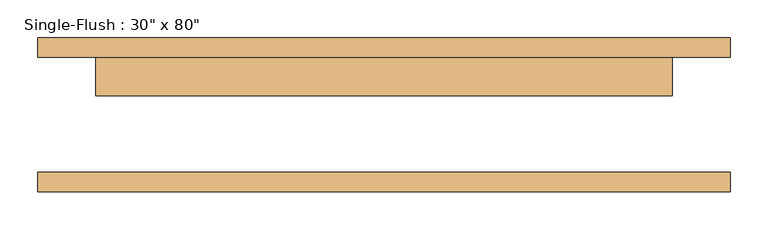
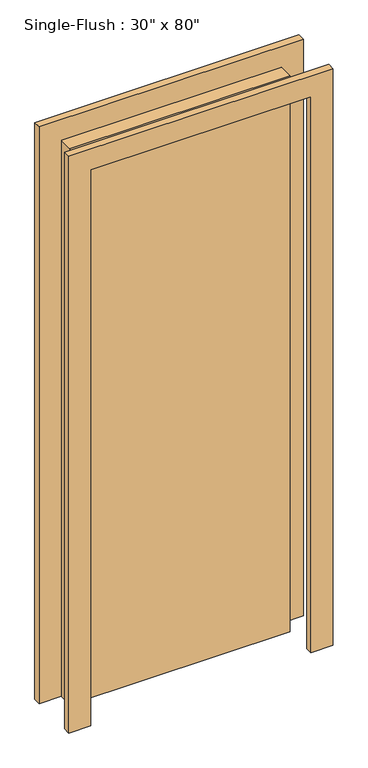
"""IFC4 building model written with IfcOpenShell, lengths in millimetres: door geometry."""

import ifcopenshell
import ifcopenshell.guid

model = None  # the IFC model being written
_history = None  # IfcOwnerHistory: only IFC2X3 demands one
_inside = {}  # id of a spatial element -> (the spatial element, [elements in it])
_under = {}  # id of a project, library or spatial element -> (it, [spatial elements below it])
_declared = {}  # id of a project -> (the project, [libraries it declares])
_typed = {}  # id of a type object -> (the type object, [elements of that type])
_made_of = {}  # id of a material, layer set ... -> (it, [elements and type objects made of it])


def new_model(schema):
    """Start an empty IFC model of exactly this schema.

    Asked for "IFC4X3", IfcOpenShell would pick the latest addendum, in which some entities
    have other attributes; the version numbers below select the first issue.
    IFC2X3 requires an IfcOwnerHistory on every rooted entity: one is made here for all.
    """
    global model, _history
    if schema == "IFC4X3":
        model = ifcopenshell.file(schema_version=(4, 3, 0, 0))
    else:
        model = ifcopenshell.file(schema=schema)
    _inside.clear()
    _under.clear()
    _declared.clear()
    _typed.clear()
    _made_of.clear()
    _history = None
    if model.schema == "IFC2X3":
        org = make("IfcOrganization", Name="unknown")
        user = make(
            "IfcPersonAndOrganization",
            ThePerson=make("IfcPerson", FamilyName="unknown"),
            TheOrganization=org,
        )
        app = make(
            "IfcApplication",
            ApplicationDeveloper=org,
            Version="unknown",
            ApplicationFullName="unknown",
            ApplicationIdentifier="unknown",
        )
        _history = make(
            "IfcOwnerHistory",
            OwningUser=user,
            OwningApplication=app,
            ChangeAction="ADDED",
            CreationDate=0,
        )
    return model


def make(cls, **values):
    """One entity of the class cls with the attributes given. An attribute that is None is left unset."""
    return model.create_entity(
        cls, **{name: value for name, value in values.items() if value is not None}
    )


def rooted(cls, **values):
    """An entity with a GlobalId (a new one), such as an element, a storey or a relation."""
    return make(cls, GlobalId=ifcopenshell.guid.new(), OwnerHistory=_history, **values)


def si_unit(unit_type, name, prefix=None):
    """IfcSIUnit, for example si_unit("LENGTHUNIT", "METRE", prefix="MILLI")."""
    return make("IfcSIUnit", UnitType=unit_type, Prefix=prefix, Name=name)


def assignment(units):
    """IfcUnitAssignment: the units of a project."""
    return None if units is None else make("IfcUnitAssignment", Units=units)


def point(xyz):
    """IfcCartesianPoint."""
    return None if xyz is None else make("IfcCartesianPoint", Coordinates=xyz)


def direction(xyz):
    """IfcDirection."""
    return None if xyz is None else make("IfcDirection", DirectionRatios=xyz)


def frame(location, z_axis=None, x_axis=None):
    """IfcAxis2Placement3D, a coordinate frame: its origin and axes. An axis left out is left unset."""
    return make(
        "IfcAxis2Placement3D",
        Location=point(location),
        Axis=direction(z_axis),
        RefDirection=direction(x_axis),
    )


def origin():
    """The frame at (0, 0, 0) with its axes left unset."""
    return frame((0.0, 0.0, 0.0))


def origin_with_axes():
    """The frame at (0, 0, 0) with the z axis (0, 0, 1) and the x axis (1, 0, 0) written out."""
    return frame((0.0, 0.0, 0.0), z_axis=(0.0, 0.0, 1.0), x_axis=(1.0, 0.0, 0.0))


def place(relative_to, where):
    """IfcLocalPlacement: puts the frame where relative to a parent placement (None: the world)."""
    return make(
        "IfcLocalPlacement", PlacementRelTo=relative_to, RelativePlacement=where
    )


def context(
    kind, dimensions, precision=None, world=None, true_north=None, identifier=None
):
    """IfcGeometricRepresentationContext, for example the 3D "Model" context."""
    return make(
        "IfcGeometricRepresentationContext",
        ContextIdentifier=identifier,
        ContextType=kind,
        CoordinateSpaceDimension=dimensions,
        Precision=precision,
        WorldCoordinateSystem=world,
        TrueNorth=true_north,
    )


def project(units=None, contexts=None):
    """IfcProject with its units and contexts."""
    return rooted(
        "IfcProject",
        Name="project",
        RepresentationContexts=contexts,
        UnitsInContext=assignment(units),
    )


def spatial(cls, under=None, at=None, **own):
    """A site, building, storey or space (cls), placed at a placement, below another one or the project."""
    s = rooted(cls, ObjectPlacement=at, **own)
    if under is not None:
        _under.setdefault(under.id(), (under, []))[1].append(s)
    return s


def polyline(points):
    """IfcPolyline through the points."""
    return make("IfcPolyline", Points=[point(p) for p in points])


def outline(outer, holes=None, kind="AREA"):
    """IfcArbitraryClosedProfileDef: a profile drawn as a closed curve; with holes, ...WithVoids."""
    if holes is None:
        return make("IfcArbitraryClosedProfileDef", ProfileType=kind, OuterCurve=outer)
    return make(
        "IfcArbitraryProfileDefWithVoids",
        ProfileType=kind,
        OuterCurve=outer,
        InnerCurves=holes,
    )


def extrude(swept, where, along, depth):
    """IfcExtrudedAreaSolid: the profile swept, set in the frame where, extruded along a direction by depth."""
    return make(
        "IfcExtrudedAreaSolid",
        SweptArea=swept,
        Position=where,
        ExtrudedDirection=direction(along),
        Depth=depth,
    )


def shape(context_of_items, identifier, shape_type, items):
    """IfcShapeRepresentation: the items that make up one representation, for example the "Body"."""
    return make(
        "IfcShapeRepresentation",
        ContextOfItems=context_of_items,
        RepresentationIdentifier=identifier,
        RepresentationType=shape_type,
        Items=items,
    )


def source(mapping_origin, context_of_items, identifier, shape_type, items):
    """IfcRepresentationMap: a shape defined once, which mapped items show again and again."""
    return make(
        "IfcRepresentationMap",
        MappingOrigin=mapping_origin,
        MappedRepresentation=shape(context_of_items, identifier, shape_type, items),
    )


def transform(
    local_origin,
    x_axis=None,
    y_axis=None,
    z_axis=None,
    scale=None,
    scale2=None,
    scale3=None,
    uniform=True,
):
    """IfcCartesianTransformationOperator3D, or its non-uniform kind. x_axis, y_axis, z_axis: its Axis1, 2, 3."""
    if uniform:
        return make(
            "IfcCartesianTransformationOperator3D",
            Axis1=direction(x_axis),
            Axis2=direction(y_axis),
            LocalOrigin=point(local_origin),
            Scale=scale,
            Axis3=direction(z_axis),
        )
    return make(
        "IfcCartesianTransformationOperator3DnonUniform",
        Axis1=direction(x_axis),
        Axis2=direction(y_axis),
        LocalOrigin=point(local_origin),
        Scale=scale,
        Axis3=direction(z_axis),
        Scale2=scale2,
        Scale3=scale3,
    )


def mapped(mapping_source, mapping_target):
    """IfcMappedItem: shows the shape of a source again, moved by a transform."""
    return make(
        "IfcMappedItem", MappingSource=mapping_source, MappingTarget=mapping_target
    )


def made_of(thing, what):
    """Note that an element or type object is made of a material, layer set ...; save() writes the relation."""
    if what is not None:
        _made_of.setdefault(what.id(), (what, []))[1].append(thing)
    return thing


def element(
    cls,
    number,
    at=None,
    inside=None,
    cuts=None,
    type_object=None,
    material=None,
    context=None,
    identifier="Body",
    shape_type=None,
    held_by="IfcProductDefinitionShape",
    body=None,
    shapes=None,
    **own,
):
    """One element of the class cls, such as IfcWall. Its Tag is "e" and its number.

    at: its placement. inside: the storey or other place that contains it. cuts: it is an
    opening in that element (IfcRelVoidsElement). A single representation is given by context,
    identifier, shape_type and body (its items); several are given by shapes. held_by: the class
    of the entity that holds the representations. save() writes the other relations.
    """
    e = rooted(cls, Tag="e%d" % number, ObjectPlacement=at, **own)
    if body is not None:
        shapes = [shape(context, identifier, shape_type, body)]
    if shapes is not None:
        e.Representation = make(held_by, Representations=shapes)
    if inside is not None:
        _inside.setdefault(inside.id(), (inside, []))[1].append(e)
    if cuts is not None:
        rooted(
            "IfcRelVoidsElement", RelatingBuildingElement=cuts, RelatedOpeningElement=e
        )
    if type_object is not None:
        _typed.setdefault(type_object.id(), (type_object, []))[1].append(e)
    return made_of(e, material)


def aggregate(whole, parts):
    """IfcRelAggregates: a whole, such as a stair, and the parts it consists of."""
    return rooted("IfcRelAggregates", RelatingObject=whole, RelatedObjects=parts)


def save(model, path):
    """Write the relations noted so far, then the file.

    IfcRelAggregates (storeys below a building ...), IfcRelContainedInSpatialStructure (elements
    in a storey), IfcRelDefinesByType, IfcRelAssociatesMaterial and IfcRelDeclares: one each for
    every whole, place, type object, material and project.
    """
    for whole, parts in _under.values():
        aggregate(whole, parts)
    for where, things in _inside.values():
        rooted(
            "IfcRelContainedInSpatialStructure",
            RelatedElements=things,
            RelatingStructure=where,
        )
    for kind, things in _typed.values():
        rooted("IfcRelDefinesByType", RelatedObjects=things, RelatingType=kind)
    for what, things in _made_of.values():
        rooted("IfcRelAssociatesMaterial", RelatedObjects=things, RelatingMaterial=what)
    for by, libraries in _declared.values():
        rooted("IfcRelDeclares", RelatingContext=by, RelatedDefinitions=libraries)
    model.write(path)


def door_059fdd7e(model_context):
    return source(origin(), model_context, "Body", "SweptSolid", [
        extrude(outline(polyline([(2108.2, -457.2), (0.0, -457.2), (0.0, -381.0), (2032.0, -381.0), (2032.0, 381.0), (0.0, 381.0), (0.0, 457.2), (2108.2, 457.2), (2108.2, -457.2)])), frame((0.0, 76.2, 0.0), z_axis=(0.0, 1.0, 0.0), x_axis=(0.0, 0.0, 1.0)), (0.0, 0.0, 1.0), 25.4),
        extrude(outline(polyline([(2108.2, 457.2), (2108.2, -457.2), (0.0, -457.2), (0.0, -381.0), (2032.0, -381.0), (2032.0, 381.0), (0.0, 381.0), (0.0, 457.2), (2108.2, 457.2)])), frame((0.0, -101.6, 0.0), z_axis=(0.0, 1.0, 0.0), x_axis=(0.0, 0.0, 1.0)), (0.0, 0.0, 1.0), 25.4),
        extrude(outline(polyline([(381.0, 25.4), (-381.0, 25.4), (-381.0, 76.2), (381.0, 76.2), (381.0, 25.4)])), origin_with_axes(), (0.0, 0.0, 1.0), 2032.0),
    ])


if __name__ == "__main__":
    model = new_model("IFC4")
    model_context = context("Model", 3, world=origin())
    ifc_project = project(units=[si_unit("LENGTHUNIT", "METRE", prefix="MILLI")], contexts=[model_context])
    site = spatial("IfcSite", under=ifc_project)
    building = spatial("IfcBuilding", under=site)
    placement = place(None, origin())
    door_shape = door_059fdd7e(model_context)
    element("IfcDoor", 1, ObjectType="Single-Flush : 30\" x 80\"", at=placement, inside=building, context=model_context, shape_type="MappedRepresentation", body=[
        mapped(door_shape, transform((0.0, 0.0, 0.0), x_axis=(1.0, 0.0, 0.0), y_axis=(0.0, 1.0, 0.0), z_axis=(0.0, 0.0, 1.0))),
    ])
    save(model, "model.ifc")

# Revit data of these elements
# Type "Single-Flush : 30\" x 80\""
#   Type Mark = "5"
#   Assembly Code = "C1020"
#   Thickness = 0' - 2"
#   Height = 6' - 8"
#   Trim Projection Ext = 0' - 1"
#   Trim Projection Int = 0' - 1"
#   Trim Width = 0' - 3"
#   Width = 2' - 6"
#   Door Material = Door - Panel
#   Frame Material = Door - Frame
#   Function = (empty or 0)
#   Wall Closure = (empty or 0)
# Element 1 (IfcDoor, "Single-Flush : 30\" x 80\"")
#   Materials on its faces: "Door - Frame", "Door - Panel"
# Materials
#   "Door - Panel": class "Wood", colour RGB 114 82 51, transparency 0
#   "Door - Frame": class "Miscellaneous", colour RGB 153 76 43, transparency 0
